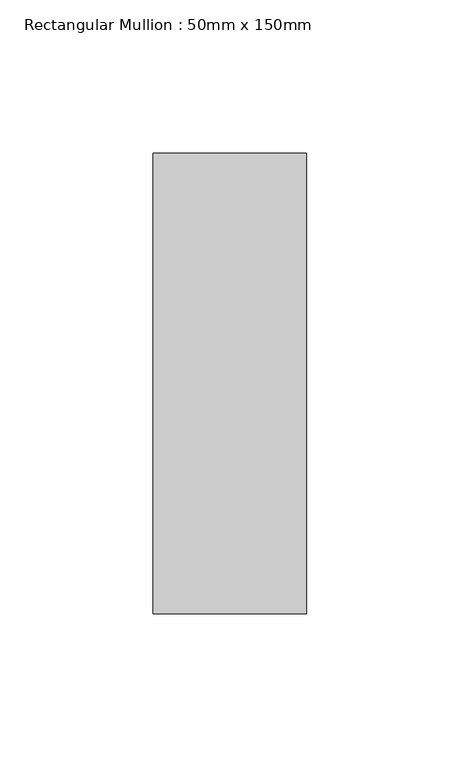
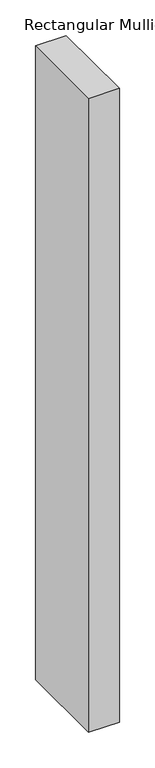
"""IFC4 building model written with IfcOpenShell, lengths in millimetres: member geometry, Rectangular Mullion : 50mm x 150mm."""

from ifc_helpers import new_model, si_unit, frame, origin, place, context, project, spatial, polyline, outline, extrude, source, transform, mapped, element, save


def rectangular_mullion_50mm_x_150mm_be4dfc7d(model_context):
    return source(origin(), model_context, "Body", "SweptSolid", [
        extrude(outline(polyline([(0.0, 75.0), (0.0, -75.0), (-50.0, -75.0), (-50.0, 75.0), (0.0, 75.0)])), frame((0.0, 0.0, -1089.0577775), z_axis=(0.0, 0.0, 1.0), x_axis=(1.0, 0.0, 0.0)), (0.0, 0.0, 1.0), 1089.0577775),
    ])


if __name__ == "__main__":
    model = new_model("IFC4")
    model_context = context("Model", 3, world=origin())
    ifc_project = project(units=[si_unit("LENGTHUNIT", "METRE", prefix="MILLI")], contexts=[model_context])
    site = spatial("IfcSite", under=ifc_project)
    building = spatial("IfcBuilding", under=site)
    placement = place(None, origin())
    rectangular_mullion_50mm_x_150mm_shape = rectangular_mullion_50mm_x_150mm_be4dfc7d(model_context)
    element("IfcMember", 1, ObjectType="Rectangular Mullion : 50mm x 150mm", at=placement, inside=building, context=model_context, shape_type="MappedRepresentation", body=[
        mapped(rectangular_mullion_50mm_x_150mm_shape, transform((0.0, 0.0, 0.0), x_axis=(1.0, 0.0, 0.0), y_axis=(0.0, 1.0, 0.0), z_axis=(0.0, 0.0, 1.0))),
    ])
    save(model, "model.ifc")

# Revit data of these elements
# Type "Rectangular Mullion : 50mm x 150mm"
#   built-in parameter 1007304 = 0.492126 (stored number, unit not read)
#   built-in parameter 1007301 = 0.082021 (stored number, unit not read)
#   built-in parameter 1007300 = 0.082021 (stored number, unit not read)
# Element 1 (IfcMember, "Rectangular Mullion : 50mm x 150mm")
#   Materials on its faces: "Aluminum"
# Materials
#   "Aluminum": class "Metal", colour RGB 247 247 247, transparency 0, Description = "Aluminum 6061", Cost = 0
